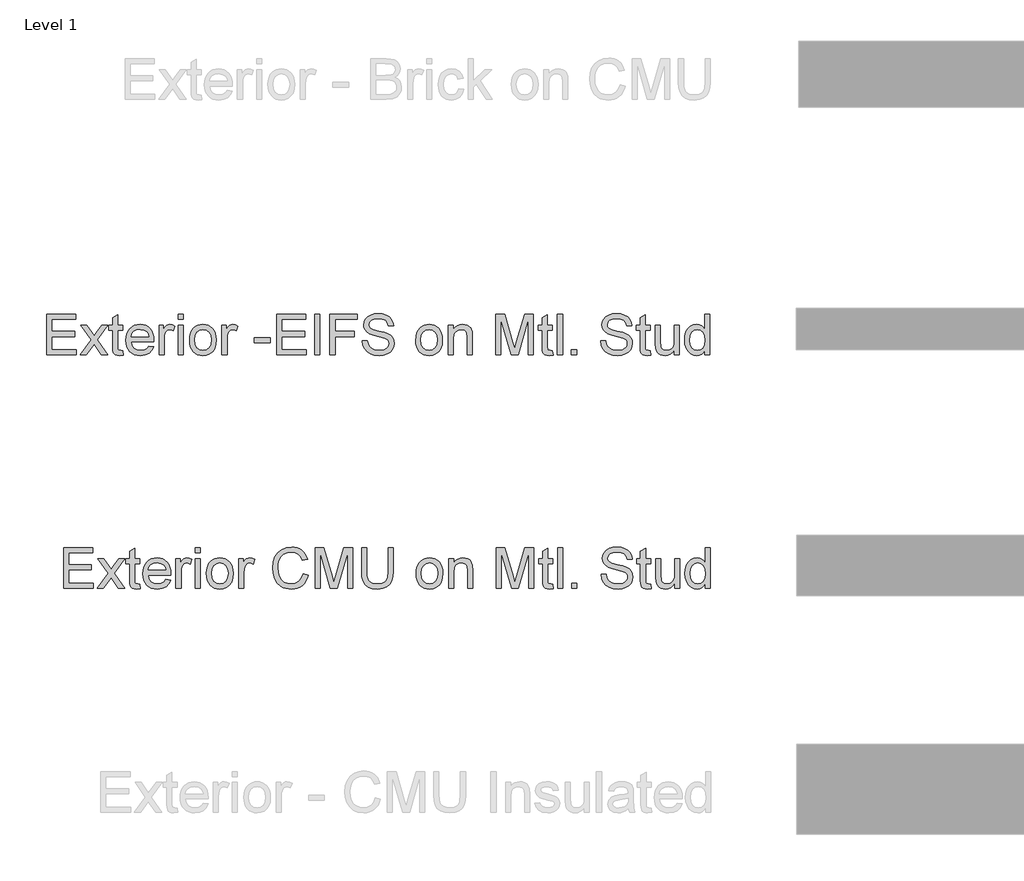
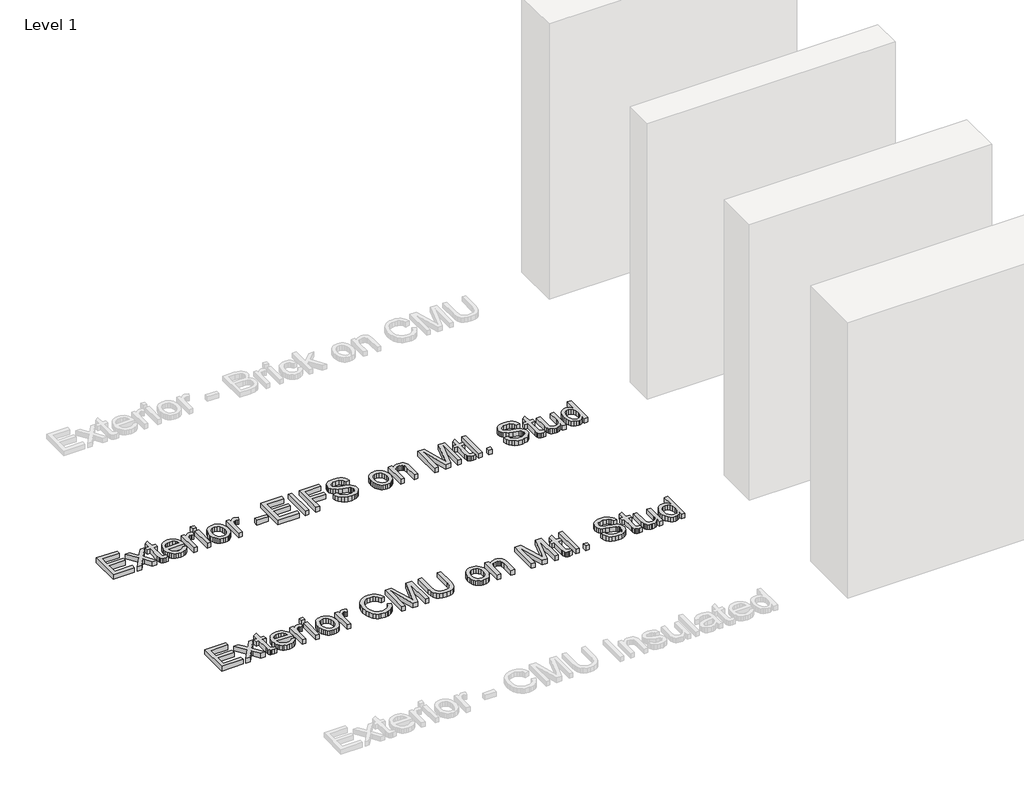
# One storey, part 21 of 42: 2 proxies.
"""IFC4 building model written with IfcOpenShell, lengths in millimetres."""

import ifcopenshell
import ifcopenshell.guid

model = None  # the IFC model being written
_history = None  # IfcOwnerHistory: only IFC2X3 demands one
_inside = {}  # id of a spatial element -> (the spatial element, [elements in it])
_under = {}  # id of a project, library or spatial element -> (it, [spatial elements below it])
_declared = {}  # id of a project -> (the project, [libraries it declares])
_typed = {}  # id of a type object -> (the type object, [elements of that type])
_made_of = {}  # id of a material, layer set ... -> (it, [elements and type objects made of it])


def new_model(schema):
    """Start an empty IFC model of exactly this schema.

    Asked for "IFC4X3", IfcOpenShell would pick the latest addendum, in which some entities
    have other attributes; the version numbers below select the first issue.
    IFC2X3 requires an IfcOwnerHistory on every rooted entity: one is made here for all.
    """
    global model, _history
    if schema == "IFC4X3":
        model = ifcopenshell.file(schema_version=(4, 3, 0, 0))
    else:
        model = ifcopenshell.file(schema=schema)
    _inside.clear()
    _under.clear()
    _declared.clear()
    _typed.clear()
    _made_of.clear()
    _history = None
    if model.schema == "IFC2X3":
        org = make("IfcOrganization", Name="unknown")
        user = make(
            "IfcPersonAndOrganization",
            ThePerson=make("IfcPerson", FamilyName="unknown"),
            TheOrganization=org,
        )
        app = make(
            "IfcApplication",
            ApplicationDeveloper=org,
            Version="unknown",
            ApplicationFullName="unknown",
            ApplicationIdentifier="unknown",
        )
        _history = make(
            "IfcOwnerHistory",
            OwningUser=user,
            OwningApplication=app,
            ChangeAction="ADDED",
            CreationDate=0,
        )
    return model


def make(cls, **values):
    """One entity of the class cls with the attributes given. An attribute that is None is left unset."""
    return model.create_entity(
        cls, **{name: value for name, value in values.items() if value is not None}
    )


def rooted(cls, **values):
    """An entity with a GlobalId (a new one), such as an element, a storey or a relation."""
    return make(cls, GlobalId=ifcopenshell.guid.new(), OwnerHistory=_history, **values)


def si_unit(unit_type, name, prefix=None):
    """IfcSIUnit, for example si_unit("LENGTHUNIT", "METRE", prefix="MILLI")."""
    return make("IfcSIUnit", UnitType=unit_type, Prefix=prefix, Name=name)


def assignment(units):
    """IfcUnitAssignment: the units of a project."""
    return None if units is None else make("IfcUnitAssignment", Units=units)


def point(xyz):
    """IfcCartesianPoint."""
    return None if xyz is None else make("IfcCartesianPoint", Coordinates=xyz)


def direction(xyz):
    """IfcDirection."""
    return None if xyz is None else make("IfcDirection", DirectionRatios=xyz)


def frame(location, z_axis=None, x_axis=None):
    """IfcAxis2Placement3D, a coordinate frame: its origin and axes. An axis left out is left unset."""
    return make(
        "IfcAxis2Placement3D",
        Location=point(location),
        Axis=direction(z_axis),
        RefDirection=direction(x_axis),
    )


def origin():
    """The frame at (0, 0, 0) with its axes left unset."""
    return frame((0.0, 0.0, 0.0))


def origin_with_axes():
    """The frame at (0, 0, 0) with the z axis (0, 0, 1) and the x axis (1, 0, 0) written out."""
    return frame((0.0, 0.0, 0.0), z_axis=(0.0, 0.0, 1.0), x_axis=(1.0, 0.0, 0.0))


def place(relative_to, where):
    """IfcLocalPlacement: puts the frame where relative to a parent placement (None: the world)."""
    return make(
        "IfcLocalPlacement", PlacementRelTo=relative_to, RelativePlacement=where
    )


def context(
    kind, dimensions, precision=None, world=None, true_north=None, identifier=None
):
    """IfcGeometricRepresentationContext, for example the 3D "Model" context."""
    return make(
        "IfcGeometricRepresentationContext",
        ContextIdentifier=identifier,
        ContextType=kind,
        CoordinateSpaceDimension=dimensions,
        Precision=precision,
        WorldCoordinateSystem=world,
        TrueNorth=true_north,
    )


def project(units=None, contexts=None):
    """IfcProject with its units and contexts."""
    return rooted(
        "IfcProject",
        Name="project",
        RepresentationContexts=contexts,
        UnitsInContext=assignment(units),
    )


def spatial(cls, under=None, at=None, **own):
    """A site, building, storey or space (cls), placed at a placement, below another one or the project."""
    s = rooted(cls, ObjectPlacement=at, **own)
    if under is not None:
        _under.setdefault(under.id(), (under, []))[1].append(s)
    return s


def polyline(points):
    """IfcPolyline through the points."""
    return make("IfcPolyline", Points=[point(p) for p in points])


def outline(outer, holes=None, kind="AREA"):
    """IfcArbitraryClosedProfileDef: a profile drawn as a closed curve; with holes, ...WithVoids."""
    if holes is None:
        return make("IfcArbitraryClosedProfileDef", ProfileType=kind, OuterCurve=outer)
    return make(
        "IfcArbitraryProfileDefWithVoids",
        ProfileType=kind,
        OuterCurve=outer,
        InnerCurves=holes,
    )


def extrude(swept, where, along, depth):
    """IfcExtrudedAreaSolid: the profile swept, set in the frame where, extruded along a direction by depth."""
    return make(
        "IfcExtrudedAreaSolid",
        SweptArea=swept,
        Position=where,
        ExtrudedDirection=direction(along),
        Depth=depth,
    )


def shape(context_of_items, identifier, shape_type, items):
    """IfcShapeRepresentation: the items that make up one representation, for example the "Body"."""
    return make(
        "IfcShapeRepresentation",
        ContextOfItems=context_of_items,
        RepresentationIdentifier=identifier,
        RepresentationType=shape_type,
        Items=items,
    )


def made_of(thing, what):
    """Note that an element or type object is made of a material, layer set ...; save() writes the relation."""
    if what is not None:
        _made_of.setdefault(what.id(), (what, []))[1].append(thing)
    return thing


def element(
    cls,
    number,
    at=None,
    inside=None,
    cuts=None,
    type_object=None,
    material=None,
    context=None,
    identifier="Body",
    shape_type=None,
    held_by="IfcProductDefinitionShape",
    body=None,
    shapes=None,
    **own,
):
    """One element of the class cls, such as IfcWall. Its Tag is "e" and its number.

    at: its placement. inside: the storey or other place that contains it. cuts: it is an
    opening in that element (IfcRelVoidsElement). A single representation is given by context,
    identifier, shape_type and body (its items); several are given by shapes. held_by: the class
    of the entity that holds the representations. save() writes the other relations.
    """
    e = rooted(cls, Tag="e%d" % number, ObjectPlacement=at, **own)
    if body is not None:
        shapes = [shape(context, identifier, shape_type, body)]
    if shapes is not None:
        e.Representation = make(held_by, Representations=shapes)
    if inside is not None:
        _inside.setdefault(inside.id(), (inside, []))[1].append(e)
    if cuts is not None:
        rooted(
            "IfcRelVoidsElement", RelatingBuildingElement=cuts, RelatedOpeningElement=e
        )
    if type_object is not None:
        _typed.setdefault(type_object.id(), (type_object, []))[1].append(e)
    return made_of(e, material)


def aggregate(whole, parts):
    """IfcRelAggregates: a whole, such as a stair, and the parts it consists of."""
    return rooted("IfcRelAggregates", RelatingObject=whole, RelatedObjects=parts)


def save(model, path):
    """Write the relations noted so far, then the file.

    IfcRelAggregates (storeys below a building ...), IfcRelContainedInSpatialStructure (elements
    in a storey), IfcRelDefinesByType, IfcRelAssociatesMaterial and IfcRelDeclares: one each for
    every whole, place, type object, material and project.
    """
    for whole, parts in _under.values():
        aggregate(whole, parts)
    for where, things in _inside.values():
        rooted(
            "IfcRelContainedInSpatialStructure",
            RelatedElements=things,
            RelatingStructure=where,
        )
    for kind, things in _typed.values():
        rooted("IfcRelDefinesByType", RelatedObjects=things, RelatingType=kind)
    for what, things in _made_of.values():
        rooted("IfcRelAssociatesMaterial", RelatedObjects=things, RelatingMaterial=what)
    for by, libraries in _declared.values():
        rooted("IfcRelDeclares", RelatingContext=by, RelatedDefinitions=libraries)
    model.write(path)


model = new_model("IFC4")

# Units and contexts
model_context = context("Model", 3, world=origin())
ifc_project = project(units=[si_unit("LENGTHUNIT", "METRE", prefix="MILLI")], contexts=[model_context])

# Site, building, storey
site = spatial("IfcSite", under=ifc_project)
building = spatial("IfcBuilding", under=site)
storey = spatial("IfcBuildingStorey", under=building, Name="Level 1", Elevation=0.0)

# Proxies
placement = place(None, origin())
element("IfcBuildingElementProxy", 1, Name="8\" Arial", ObjectType="8\" Arial", at=placement, inside=storey, context=model_context, shape_type="SweptSolid", body=[
    extrude(outline(polyline([(-4947.8204777, 6427.3124108), (-4947.8204777, 6731.8795049), (-4728.9128788, 6731.8795049), (-4728.9128788, 6693.8086181), (-4909.7495909, 6693.8086181), (-4909.7495909, 6603.390262), (-4738.4306005, 6603.390262), (-4738.4306005, 6565.3193753), (-4909.7495909, 6565.3193753), (-4909.7495909, 6465.3832975), (-4724.154018, 6465.3832975), (-4724.154018, 6427.3124108), (-4947.8204777, 6427.3124108)])), origin_with_axes(), (0.0, 0.0, 1.0), 50.8),
    extrude(outline(polyline([(-4695.6008529, 6427.3124108), (-4614.2540754, 6539.7404982), (-4690.8419921, 6650.9788705), (-4645.0379564, 6650.9788705), (-4608.0824277, 6597.441686), (-4590.8315571, 6572.1602377), (-4575.8857598, 6592.8315395), (-4533.7995842, 6650.9788705), (-4487.9955486, 6650.9788705), (-4568.4500397, 6539.7404982), (-4490.9698366, 6427.3124108), (-4536.7738722, 6427.3124108), (-4583.3958371, 6494.9031062), (-4591.9469151, 6507.2464015), (-4649.7968173, 6427.3124108), (-4695.6008529, 6427.3124108)])), origin_with_axes(), (0.0, 0.0, 1.0), 50.8),
    extrude(outline(polyline([(-4376.7571763, 6459.0629355), (-4371.9983155, 6426.1970528), (-4400.4771233, 6422.5535499), (-4418.7504054, 6424.1336405), (-4432.3763624, 6428.873912), (-4442.0056199, 6436.179507), (-4448.2888034, 6445.4555678), (-4451.7464132, 6461.386598), (-4452.8989498, 6488.6571014), (-4452.8989498, 6612.9079837), (-4481.4521149, 6612.9079837), (-4481.4521149, 6650.9788705), (-4452.8989498, 6650.9788705), (-4452.8989498, 6705.3339842), (-4414.8280631, 6727.7155016), (-4414.8280631, 6650.9788705), (-4376.7571763, 6650.9788705), (-4376.7571763, 6612.9079837), (-4414.8280631, 6612.9079837), (-4414.8280631, 6489.7724594), (-4412.8204187, 6470.1421584), (-4406.3141636, 6463.1897601), (-4393.3388321, 6460.6244367), (-4376.7571763, 6459.0629355)])), origin_with_axes(), (0.0, 0.0, 1.0), 50.8),
    extrude(outline(polyline([(-4182.0900249, 6493.9364626), (-4144.7627101, 6489.1776018), (-4158.2120688, 6461.0519906), (-4179.6734159, 6440.0274921), (-4208.6634295, 6426.9220355), (-4244.6987879, 6422.5535499), (-4268.3211411, 6424.4380402), (-4289.3688762, 6430.0915112), (-4307.8419932, 6439.5139627), (-4323.7404922, 6452.7053948), (-4336.5252834, 6469.2986689), (-4345.6572771, 6488.9266462), (-4351.1364734, 6511.5893268), (-4352.9628721, 6537.2867106), (-4351.1178841, 6563.8554679), (-4345.5829199, 6587.2733388), (-4336.3579797, 6607.5403233), (-4323.4430634, 6624.6564214), (-4307.5863904, 6638.2544945), (-4289.5361799, 6647.9674039), (-4269.292432, 6653.7951495), (-4246.8551467, 6655.7377313), (-4225.1405204, 6653.7997968), (-4205.5032485, 6647.9859932), (-4187.9433308, 6638.2963204), (-4172.4607674, 6624.7307786), (-4159.8223669, 6607.6518591), (-4150.794938, 6587.4220532), (-4145.3784807, 6564.0413609), (-4143.5729949, 6537.5097822), (-4143.7960665, 6527.2484885), (-4314.8919853, 6527.2484885), (-4308.3020784, 6498.7510914), (-4292.9937897, 6477.8009501), (-4270.9004065, 6464.918565), (-4243.9552159, 6460.6244367), (-4223.6928787, 6462.6134918), (-4206.6279011, 6468.5806572), (-4192.7602832, 6478.8977188), (-4182.0900249, 6493.9364626)]), holes=[polyline([(-4314.8919853, 6565.3193753), (-4181.6438817, 6565.3193753), (-4186.7931178, 6585.4329981), (-4196.8871078, 6599.8211164), (-4219.0827322, 6613.2054125), (-4247.0038611, 6617.6668446), (-4272.66639, 6614.1069936), (-4293.8860761, 6603.4274406), (-4308.6366858, 6586.7807223), (-4314.8919853, 6565.3193753)])]), origin_with_axes(), (0.0, 0.0, 1.0), 50.8),
    extrude(outline(polyline([(-4105.5021082, 6427.3124108), (-4105.5021082, 6650.9788705), (-4072.1900823, 6650.9788705), (-4072.1900823, 6617.8899162), (-4059.8839655, 6637.074074), (-4048.5444924, 6648.3763685), (-4037.1678407, 6653.8973906), (-4024.7501882, 6655.7377313), (-4005.789102, 6652.8006219), (-3986.530587, 6643.9892936), (-3999.2456684, 6609.8593385), (-4012.6299645, 6615.7149681), (-4026.0142606, 6617.6668446), (-4037.3816177, 6615.7893253), (-4047.5406702, 6610.1567673), (-4055.7478462, 6601.1967246), (-4061.2595737, 6589.3367511), (-4065.8883095, 6568.0705917), (-4067.4312214, 6544.8711451), (-4067.4312214, 6427.3124108), (-4105.5021082, 6427.3124108)])), origin_with_axes(), (0.0, 0.0, 1.0), 50.8),
    extrude(outline(polyline([(-3962.7362828, 6693.8086181), (-3962.7362828, 6731.8795049), (-3924.6653961, 6731.8795049), (-3924.6653961, 6693.8086181), (-3962.7362828, 6693.8086181)])), origin_with_axes(), (0.0, 0.0, 1.0), 50.8),
    extrude(outline(polyline([(-3962.7362828, 6427.3124108), (-3962.7362828, 6650.9788705), (-3924.6653961, 6650.9788705), (-3924.6653961, 6427.3124108), (-3962.7362828, 6427.3124108)])), origin_with_axes(), (0.0, 0.0, 1.0), 50.8),
    extrude(outline(polyline([(-3877.0767876, 6539.1456406), (-3875.0180226, 6568.1124176), (-3868.8417276, 6593.0732004), (-3858.5479027, 6614.0279891), (-3844.1365477, 6630.9767835), (-3829.6275989, 6641.8096982), (-3813.6129168, 6649.5474944), (-3796.0925014, 6654.1901721), (-3777.0663527, 6655.7377313), (-3756.0627671, 6653.853241), (-3737.0714733, 6648.1997701), (-3720.0924713, 6638.7773186), (-3705.125761, 6625.5858865), (-3692.9102671, 6609.0716169), (-3684.1849143, 6589.6806532), (-3678.9497027, 6567.4129952), (-3677.2046321, 6542.2686431), (-3680.290456, 6503.807381), (-3689.5479274, 6474.5292332), (-3704.7075017, 6452.6031537), (-3725.499634, 6436.1980963), (-3750.1955193, 6425.9646865), (-3777.0663527, 6422.5535499), (-3798.3766617, 6424.4310693), (-3817.5445538, 6430.0636272), (-3834.5700291, 6439.4512238), (-3849.4530876, 6452.593859), (-3861.5384563, 6469.2684613), (-3870.1708626, 6489.251959), (-3875.3503064, 6512.5443521), (-3877.0767876, 6539.1456406)]), holes=[polyline([(-3839.0059009, 6539.2199978), (-3834.6002367, 6504.76473), (-3821.3832443, 6480.2175591), (-3801.4926931, 6465.5227173), (-3777.0663527, 6460.6244367), (-3752.751548, 6465.5506012), (-3732.8981755, 6480.3290949), (-3719.681183, 6505.2015785), (-3715.2755189, 6540.409713), (-3719.709067, 6573.8611587), (-3733.0097113, 6598.0737222), (-3752.8909678, 6612.768564), (-3777.0663527, 6617.6668446), (-3801.4926931, 6612.7871533), (-3821.3832443, 6598.1480794), (-3834.6002367, 6573.6566764), (-3839.0059009, 6539.2199978)])]), origin_with_axes(), (0.0, 0.0, 1.0), 50.8),
    extrude(outline(polyline([(-3634.3748845, 6427.3124108), (-3634.3748845, 6650.9788705), (-3601.0628586, 6650.9788705), (-3601.0628586, 6617.8899162), (-3588.7567419, 6637.074074), (-3577.4172688, 6648.3763685), (-3566.0406171, 6653.8973906), (-3553.6229646, 6655.7377313), (-3534.6618784, 6652.8006219), (-3515.4033634, 6643.9892936), (-3528.1184447, 6609.8593385), (-3541.5027409, 6615.7149681), (-3554.887037, 6617.6668446), (-3566.254394, 6615.7893253), (-3576.4134466, 6610.1567673), (-3584.6206226, 6601.1967246), (-3590.1323501, 6589.3367511), (-3594.7610859, 6568.0705917), (-3596.3039978, 6544.8711451), (-3596.3039978, 6427.3124108), (-3634.3748845, 6427.3124108)])), origin_with_axes(), (0.0, 0.0, 1.0), 50.8),
    extrude(outline(polyline([(-3391.6729814, 6517.7307668), (-3391.6729814, 6555.8016536), (-3272.7014603, 6555.8016536), (-3272.7014603, 6517.7307668), (-3391.6729814, 6517.7307668)])), origin_with_axes(), (0.0, 0.0, 1.0), 50.8),
    extrude(outline(polyline([(-3225.1128519, 6427.3124108), (-3225.1128519, 6731.8795049), (-3006.205253, 6731.8795049), (-3006.205253, 6693.8086181), (-3187.0419651, 6693.8086181), (-3187.0419651, 6603.390262), (-3015.7229747, 6603.390262), (-3015.7229747, 6565.3193753), (-3187.0419651, 6565.3193753), (-3187.0419651, 6465.3832975), (-3001.4463922, 6465.3832975), (-3001.4463922, 6427.3124108), (-3225.1128519, 6427.3124108)])), origin_with_axes(), (0.0, 0.0, 1.0), 50.8),
    extrude(outline(polyline([(-2939.5812012, 6427.3124108), (-2939.5812012, 6731.8795049), (-2901.5103144, 6731.8795049), (-2901.5103144, 6427.3124108), (-2939.5812012, 6427.3124108)])), origin_with_axes(), (0.0, 0.0, 1.0), 50.8),
    extrude(outline(polyline([(-2825.3685409, 6427.3124108), (-2825.3685409, 6731.8795049), (-2620.7375246, 6731.8795049), (-2620.7375246, 6693.8086181), (-2787.2976542, 6693.8086181), (-2787.2976542, 6603.390262), (-2644.5318288, 6603.390262), (-2644.5318288, 6565.3193753), (-2787.2976542, 6565.3193753), (-2787.2976542, 6427.3124108), (-2825.3685409, 6427.3124108)])), origin_with_axes(), (0.0, 0.0, 1.0), 50.8),
    extrude(outline(polyline([(-2582.6666378, 6532.0073494), (-2544.5957511, 6532.0073494), (-2540.2272655, 6510.8806097), (-2532.3268129, 6493.899284), (-2520.0021069, 6480.4220414), (-2502.3608611, 6469.807551), (-2480.7972729, 6462.9202153), (-2456.7055398, 6460.6244367), (-2435.4951483, 6462.3625363), (-2416.9244375, 6467.576835), (-2401.876399, 6475.8304842), (-2391.2340246, 6486.6866355), (-2384.9043679, 6499.1507613), (-2382.7944823, 6512.228334), (-2384.3745729, 6524.9712993), (-2389.1148444, 6535.9854596), (-2398.7441019, 6545.3823508), (-2414.9911502, 6553.2735088), (-2470.4244434, 6567.8103415), (-2506.8129985, 6577.4303043), (-2530.0960969, 6586.5855347), (-2549.0478885, 6599.3935625), (-2562.4786578, 6614.9156281), (-2570.4813516, 6632.8171242), (-2573.1489161, 6652.7634433), (-2569.8493154, 6675.0613089), (-2559.950513, 6695.8534411), (-2543.7127593, 6713.4760977), (-2521.3963044, 6726.2655362), (-2494.6091229, 6734.0451583), (-2464.9591891, 6736.6383657), (-2432.8368784, 6733.9243279), (-2404.7298565, 6725.7822144), (-2381.6419457, 6712.379329), (-2364.5769682, 6693.8829753), (-2353.7765848, 6671.44569), (-2349.4824564, 6646.2200096), (-2387.5533432, 6646.2200096), (-2394.5429201, 6668.9361345), (-2409.1169314, 6685.3318972), (-2431.8888241, 6695.2585835), (-2463.4720451, 6698.5674789), (-2495.7988381, 6695.2957621), (-2517.9758732, 6685.4806116), (-2530.8024903, 6671.0367254), (-2535.0780294, 6653.8788013), (-2532.0479734, 6639.2490221), (-2522.9578057, 6627.4819951), (-2501.4685747, 6616.9604512), (-2460.7951859, 6606.2158357), (-2418.8205461, 6596.0103099), (-2393.427562, 6587.1060351), (-2371.7245541, 6573.2941851), (-2356.5835691, 6556.2477968), (-2347.688589, 6536.1527633), (-2344.7235956, 6513.1949776), (-2348.1347322, 6489.7259861), (-2358.3681419, 6467.6511922), (-2375.0055656, 6448.6529274), (-2397.6287439, 6434.4135234), (-2424.8341847, 6425.5185433), (-2455.2183958, 6422.5535499), (-2492.5178266, 6425.7509096), (-2523.2180559, 6435.3429885), (-2547.6722802, 6451.3669652), (-2566.2336965, 6473.8600184), (-2578.1494379, 6501.2606469), (-2582.6666378, 6532.0073494)])), origin_with_axes(), (0.0, 0.0, 1.0), 50.8),
    extrude(outline(polyline([(-2182.9223269, 6539.1456406), (-2180.8635619, 6568.1124176), (-2174.6872669, 6593.0732004), (-2164.3934419, 6614.0279891), (-2149.9820869, 6630.9767835), (-2135.4731382, 6641.8096982), (-2119.4584561, 6649.5474944), (-2101.9380406, 6654.1901721), (-2082.9118919, 6655.7377313), (-2061.9083064, 6653.853241), (-2042.9170126, 6648.1997701), (-2025.9380105, 6638.7773186), (-2010.9713002, 6625.5858865), (-1998.7558064, 6609.0716169), (-1990.0304536, 6589.6806532), (-1984.7952419, 6567.4129952), (-1983.0501714, 6542.2686431), (-1986.1359952, 6503.807381), (-1995.3934667, 6474.5292332), (-2010.553041, 6452.6031537), (-2031.3451732, 6436.1980963), (-2056.0410585, 6425.9646865), (-2082.9118919, 6422.5535499), (-2104.2222009, 6424.4310693), (-2123.390093, 6430.0636272), (-2140.4155683, 6439.4512238), (-2155.2986268, 6452.593859), (-2167.3839956, 6469.2684613), (-2176.0164018, 6489.251959), (-2181.1958456, 6512.5443521), (-2182.9223269, 6539.1456406)]), holes=[polyline([(-2144.8514401, 6539.2199978), (-2140.445776, 6504.76473), (-2127.2287835, 6480.2175591), (-2107.3382323, 6465.5227173), (-2082.9118919, 6460.6244367), (-2058.5970873, 6465.5506012), (-2038.7437147, 6480.3290949), (-2025.5267223, 6505.2015785), (-2021.1210581, 6540.409713), (-2025.5546062, 6573.8611587), (-2038.8552505, 6598.0737222), (-2058.736507, 6612.768564), (-2082.9118919, 6617.6668446), (-2107.3382323, 6612.7871533), (-2127.2287835, 6598.1480794), (-2140.445776, 6573.6566764), (-2144.8514401, 6539.2199978)])]), origin_with_axes(), (0.0, 0.0, 1.0), 50.8),
    extrude(outline(polyline([(-1940.2204238, 6427.3124108), (-1940.2204238, 6650.9788705), (-1902.149537, 6650.9788705), (-1902.149537, 6619.7488462), (-1888.9232499, 6635.4939834), (-1873.0386929, 6646.74051), (-1854.495866, 6653.488426), (-1833.2947692, 6655.7377313), (-1814.5288706, 6653.9252746), (-1797.3430626, 6648.4879043), (-1783.0107122, 6640.1041299), (-1772.8051864, 6629.4524609), (-1761.3913561, 6601.4569748), (-1759.3837117, 6564.6501605), (-1759.3837117, 6427.3124108), (-1797.4545984, 6427.3124108), (-1797.4545984, 6559.5195136), (-1801.8416733, 6593.2033255), (-1807.9110798, 6603.232253), (-1817.3451496, 6611.0118751), (-1829.4374894, 6616.0031022), (-1843.4817057, 6617.6668446), (-1865.7795712, 6613.9303952), (-1884.7871307, 6602.7210472), (-1892.3831834, 6593.5704642), (-1897.8089354, 6581.0645125), (-1902.149537, 6545.9865031), (-1902.149537, 6427.3124108), (-1940.2204238, 6427.3124108)])), origin_with_axes(), (0.0, 0.0, 1.0), 50.8),
    extrude(outline(polyline([(-1583.3058604, 6427.3124108), (-1583.3058604, 6731.8795049), (-1517.7971666, 6731.8795049), (-1455.4858324, 6517.2102664), (-1442.9194655, 6472.3728744), (-1429.3120978, 6520.9281265), (-1368.0417644, 6731.8795049), (-1302.5330706, 6731.8795049), (-1302.5330706, 6427.3124108), (-1340.6039573, 6427.3124108), (-1340.6039573, 6693.8086181), (-1417.1175168, 6427.3124108), (-1468.7214141, 6427.3124108), (-1545.2349737, 6693.8086181), (-1545.2349737, 6427.3124108), (-1583.3058604, 6427.3124108)])), origin_with_axes(), (0.0, 0.0, 1.0), 50.8),
    extrude(outline(polyline([(-1159.7672452, 6459.0629355), (-1155.0083844, 6426.1970528), (-1183.4871922, 6422.5535499), (-1201.7604743, 6424.1336405), (-1215.3864313, 6428.873912), (-1225.0156888, 6436.179507), (-1231.2988723, 6445.4555678), (-1234.7564821, 6461.386598), (-1235.9090187, 6488.6571014), (-1235.9090187, 6612.9079837), (-1264.4621838, 6612.9079837), (-1264.4621838, 6650.9788705), (-1235.9090187, 6650.9788705), (-1235.9090187, 6705.3339842), (-1197.838132, 6727.7155016), (-1197.838132, 6650.9788705), (-1159.7672452, 6650.9788705), (-1159.7672452, 6612.9079837), (-1197.838132, 6612.9079837), (-1197.838132, 6489.7724594), (-1195.8304876, 6470.1421584), (-1189.3242325, 6463.1897601), (-1176.348901, 6460.6244367), (-1159.7672452, 6459.0629355)])), origin_with_axes(), (0.0, 0.0, 1.0), 50.8),
    extrude(outline(polyline([(-1121.6963585, 6427.3124108), (-1121.6963585, 6731.8795049), (-1083.6254717, 6731.8795049), (-1083.6254717, 6427.3124108), (-1121.6963585, 6427.3124108)])), origin_with_axes(), (0.0, 0.0, 1.0), 50.8),
    extrude(outline(polyline([(-1017.0014199, 6427.3124108), (-1017.0014199, 6465.3832975), (-978.9305331, 6465.3832975), (-978.9305331, 6427.3124108), (-1017.0014199, 6427.3124108)])), origin_with_axes(), (0.0, 0.0, 1.0), 50.8),
    extrude(outline(polyline([(-798.093821, 6532.0073494), (-760.0229343, 6532.0073494), (-755.6544487, 6510.8806097), (-747.7539961, 6493.899284), (-735.4292901, 6480.4220414), (-717.7880443, 6469.807551), (-696.2244561, 6462.9202153), (-672.132723, 6460.6244367), (-650.9223315, 6462.3625363), (-632.3516207, 6467.576835), (-617.3035822, 6475.8304842), (-606.6612078, 6486.6866355), (-600.3315511, 6499.1507613), (-598.2216655, 6512.228334), (-599.801756, 6524.9712993), (-604.5420276, 6535.9854596), (-614.1712851, 6545.3823508), (-630.4183334, 6553.2735088), (-685.8516266, 6567.8103415), (-722.2401817, 6577.4303043), (-745.5232801, 6586.5855347), (-764.4750717, 6599.3935625), (-777.905841, 6614.9156281), (-785.9085348, 6632.8171242), (-788.5760993, 6652.7634433), (-785.2764985, 6675.0613089), (-775.3776962, 6695.8534411), (-759.1399425, 6713.4760977), (-736.8234876, 6726.2655362), (-710.0363061, 6734.0451583), (-680.3863723, 6736.6383657), (-648.2640616, 6733.9243279), (-620.1570397, 6725.7822144), (-597.0691289, 6712.379329), (-580.0041514, 6693.8829753), (-569.203768, 6671.44569), (-564.9096396, 6646.2200096), (-602.9805264, 6646.2200096), (-609.9701032, 6668.9361345), (-624.5441146, 6685.3318972), (-647.3160073, 6695.2585835), (-678.8992283, 6698.5674789), (-711.2260213, 6695.2957621), (-733.4030564, 6685.4806116), (-746.2296735, 6671.0367254), (-750.5052126, 6653.8788013), (-747.4751566, 6639.2490221), (-738.3849889, 6627.4819951), (-716.8957579, 6616.9604512), (-676.2223691, 6606.2158357), (-634.2477293, 6596.0103099), (-608.8547452, 6587.1060351), (-587.1517373, 6573.2941851), (-572.0107523, 6556.2477968), (-563.1157722, 6536.1527633), (-560.1507788, 6513.1949776), (-563.5619154, 6489.7259861), (-573.7953251, 6467.6511922), (-590.4327488, 6448.6529274), (-613.0559271, 6434.4135234), (-640.2613679, 6425.5185433), (-670.645579, 6422.5535499), (-707.9450098, 6425.7509096), (-738.6452391, 6435.3429885), (-763.0994634, 6451.3669652), (-781.6608797, 6473.8600184), (-793.5766211, 6501.2606469), (-798.093821, 6532.0073494)])), origin_with_axes(), (0.0, 0.0, 1.0), 50.8),
    extrude(outline(polyline([(-426.9026751, 6459.0629355), (-422.1438143, 6426.1970528), (-450.6226221, 6422.5535499), (-468.8959042, 6424.1336405), (-482.5218612, 6428.873912), (-492.1511187, 6436.179507), (-498.4343022, 6445.4555678), (-501.891912, 6461.386598), (-503.0444486, 6488.6571014), (-503.0444486, 6612.9079837), (-531.5976137, 6612.9079837), (-531.5976137, 6650.9788705), (-503.0444486, 6650.9788705), (-503.0444486, 6705.3339842), (-464.9735619, 6727.7155016), (-464.9735619, 6650.9788705), (-426.9026751, 6650.9788705), (-426.9026751, 6612.9079837), (-464.9735619, 6612.9079837), (-464.9735619, 6489.7724594), (-462.9659175, 6470.1421584), (-456.4596624, 6463.1897601), (-443.4843309, 6460.6244367), (-426.9026751, 6459.0629355)])), origin_with_axes(), (0.0, 0.0, 1.0), 50.8),
    extrude(outline(polyline([(-246.065963, 6427.3124108), (-246.065963, 6465.7550835), (-259.8406344, 6446.8544126), (-275.8832005, 6433.3539333), (-294.1936612, 6425.2536458), (-314.7720165, 6422.5535499), (-333.3148434, 6424.4496586), (-350.5750086, 6430.1379844), (-365.0560734, 6438.6890625), (-375.2615992, 6449.1734278), (-382.1303456, 6461.9070984), (-386.6010723, 6477.2060925), (-388.8317884, 6512.60012), (-388.8317884, 6650.9788705), (-350.7609016, 6650.9788705), (-350.7609016, 6530.5202054), (-348.4558284, 6491.7057466), (-342.9069223, 6478.758299), (-333.3984952, 6468.9152646), (-320.5625835, 6462.6971437), (-305.0312232, 6460.6244367), (-288.6075765, 6462.7436169), (-273.2435199, 6469.1011576), (-260.5749118, 6479.1114957), (-252.2376107, 6492.1890684), (-247.6088749, 6510.0998591), (-246.065963, 6534.6098514), (-246.065963, 6650.9788705), (-207.9950763, 6650.9788705), (-207.9950763, 6427.3124108), (-246.065963, 6427.3124108)])), origin_with_axes(), (0.0, 0.0, 1.0), 50.8),
    extrude(outline(polyline([(-17.6406425, 6427.3124108), (-17.6406425, 6463.2269387), (-29.0312361, 6445.4323311), (-42.8291442, 6432.7218971), (-59.0343666, 6425.0956367), (-77.6469034, 6422.5535499), (-102.2591369, 6426.2342314), (-124.7893687, 6437.2762757), (-143.8619907, 6454.9082269), (-158.1013946, 6478.3586291), (-166.9684908, 6506.6794279), (-169.9241895, 6538.922569), (-167.200857, 6570.7660402), (-159.0308596, 6599.5236876), (-145.4234919, 6623.5596527), (-126.3880485, 6641.2380772), (-103.3652002, 6652.1128178), (-77.7956178, 6655.7377313), (-59.1691391, 6653.144524), (-42.6990191, 6645.3649018), (-28.7384547, 6633.4398658), (-17.6406425, 6618.4104166), (-17.6406425, 6731.8795049), (20.4302443, 6731.8795049), (20.4302443, 6427.3124108), (-17.6406425, 6427.3124108)]), holes=[polyline([(-131.8533027, 6539.0712834), (-127.5591744, 6504.6346049), (-114.6767894, 6480.1432019), (-95.9573641, 6465.504128), (-74.152115, 6460.6244367), (-52.3561605, 6465.2810564), (-34.1107624, 6479.2509155), (-21.7581725, 6502.7942641), (-17.6406425, 6536.1713526), (-21.8325297, 6572.6621489), (-34.4081912, 6597.9621864), (-53.1183219, 6612.74068), (-75.7136162, 6617.6668446), (-97.7419369, 6612.9358677), (-115.7921474, 6598.742937), (-127.8380139, 6574.3630698), (-131.8533027, 6539.0712834)])]), origin_with_axes(), (0.0, 0.0, 1.0), 50.8),
])
element("IfcBuildingElementProxy", 2, Name="8\" Arial", ObjectType="8\" Arial", at=placement, inside=storey, context=model_context, shape_type="SweptSolid", body=[
    extrude(outline(polyline([(-4820.8204777, 4678.9650607), (-4820.8204777, 4983.5321548), (-4601.9128788, 4983.5321548), (-4601.9128788, 4945.461268), (-4782.7495909, 4945.461268), (-4782.7495909, 4855.042912), (-4611.4306005, 4855.042912), (-4611.4306005, 4816.9720252), (-4782.7495909, 4816.9720252), (-4782.7495909, 4717.0359475), (-4597.154018, 4717.0359475), (-4597.154018, 4678.9650607), (-4820.8204777, 4678.9650607)])), origin_with_axes(), (0.0, 0.0, 1.0), 50.8),
    extrude(outline(polyline([(-4568.6008529, 4678.9650607), (-4487.2540754, 4791.3931482), (-4563.8419921, 4902.6315204), (-4518.0379564, 4902.6315204), (-4481.0824277, 4849.0943359), (-4463.8315571, 4823.8128877), (-4448.8857598, 4844.4841895), (-4406.7995842, 4902.6315204), (-4360.9955486, 4902.6315204), (-4441.4500397, 4791.3931482), (-4363.9698366, 4678.9650607), (-4409.7738722, 4678.9650607), (-4456.3958371, 4746.5557562), (-4464.9469151, 4758.8990515), (-4522.7968173, 4678.9650607), (-4568.6008529, 4678.9650607)])), origin_with_axes(), (0.0, 0.0, 1.0), 50.8),
    extrude(outline(polyline([(-4249.7571763, 4710.7155854), (-4244.9983155, 4677.8497027), (-4273.4771233, 4674.2061999), (-4291.7504054, 4675.7862904), (-4305.3763624, 4680.526562), (-4315.0056199, 4687.8321569), (-4321.2888034, 4697.1082177), (-4324.7464132, 4713.039248), (-4325.8989498, 4740.3097513), (-4325.8989498, 4864.5606337), (-4354.4521149, 4864.5606337), (-4354.4521149, 4902.6315204), (-4325.8989498, 4902.6315204), (-4325.8989498, 4956.9866342), (-4287.8280631, 4979.3681516), (-4287.8280631, 4902.6315204), (-4249.7571763, 4902.6315204), (-4249.7571763, 4864.5606337), (-4287.8280631, 4864.5606337), (-4287.8280631, 4741.4251093), (-4285.8204187, 4721.7948083), (-4279.3141636, 4714.8424101), (-4266.3388321, 4712.2770867), (-4249.7571763, 4710.7155854)])), origin_with_axes(), (0.0, 0.0, 1.0), 50.8),
    extrude(outline(polyline([(-4055.0900249, 4745.5891126), (-4017.7627101, 4740.8302517), (-4031.2120688, 4712.7046406), (-4052.6734159, 4691.6801421), (-4081.6634295, 4678.5746854), (-4117.6987879, 4674.2061999), (-4141.3211411, 4676.0906902), (-4162.3688762, 4681.7441611), (-4180.8419932, 4691.1666126), (-4196.7404922, 4704.3580448), (-4209.5252834, 4720.9513188), (-4218.6572771, 4740.5792962), (-4224.1364734, 4763.2419767), (-4225.9628721, 4788.9393606), (-4224.1178841, 4815.5081179), (-4218.5829199, 4838.9259887), (-4209.3579797, 4859.1929733), (-4196.4430634, 4876.3090714), (-4180.5863904, 4889.9071445), (-4162.5361799, 4899.6200538), (-4142.292432, 4905.4477994), (-4119.8551467, 4907.3903813), (-4098.1405204, 4905.4524467), (-4078.5032485, 4899.6386431), (-4060.9433308, 4889.9489704), (-4045.4607674, 4876.3834286), (-4032.8223669, 4859.3045091), (-4023.794938, 4839.0747031), (-4018.3784807, 4815.6940109), (-4016.5729949, 4789.1624322), (-4016.7960665, 4778.9011385), (-4187.8919853, 4778.9011385), (-4181.3020784, 4750.4037413), (-4165.9937897, 4729.4536), (-4143.9004065, 4716.571215), (-4116.9552159, 4712.2770867), (-4096.6928787, 4714.2661418), (-4079.6279011, 4720.2333071), (-4065.7602832, 4730.5503687), (-4055.0900249, 4745.5891126)]), holes=[polyline([(-4187.8919853, 4816.9720252), (-4054.6438817, 4816.9720252), (-4059.7931178, 4837.085648), (-4069.8871078, 4851.4737664), (-4092.0827322, 4864.8580625), (-4120.0038611, 4869.3194945), (-4145.66639, 4865.7596435), (-4166.8860761, 4855.0800906), (-4181.6366858, 4838.4333723), (-4187.8919853, 4816.9720252)])]), origin_with_axes(), (0.0, 0.0, 1.0), 50.8),
    extrude(outline(polyline([(-3978.5021082, 4678.9650607), (-3978.5021082, 4902.6315204), (-3945.1900823, 4902.6315204), (-3945.1900823, 4869.5425661), (-3932.8839655, 4888.7267239), (-3921.5444924, 4900.0290184), (-3910.1678407, 4905.5500406), (-3897.7501882, 4907.3903813), (-3878.789102, 4904.4532719), (-3859.530587, 4895.6419436), (-3872.2456684, 4861.5119885), (-3885.6299645, 4867.367618), (-3899.0142606, 4869.3194945), (-3910.3816177, 4867.4419752), (-3920.5406702, 4861.8094173), (-3928.7478462, 4852.8493746), (-3934.2595737, 4840.9894011), (-3938.8883095, 4819.7232417), (-3940.4312214, 4796.523795), (-3940.4312214, 4678.9650607), (-3978.5021082, 4678.9650607)])), origin_with_axes(), (0.0, 0.0, 1.0), 50.8),
    extrude(outline(polyline([(-3835.7362828, 4945.461268), (-3835.7362828, 4983.5321548), (-3797.6653961, 4983.5321548), (-3797.6653961, 4945.461268), (-3835.7362828, 4945.461268)])), origin_with_axes(), (0.0, 0.0, 1.0), 50.8),
    extrude(outline(polyline([(-3835.7362828, 4678.9650607), (-3835.7362828, 4902.6315204), (-3797.6653961, 4902.6315204), (-3797.6653961, 4678.9650607), (-3835.7362828, 4678.9650607)])), origin_with_axes(), (0.0, 0.0, 1.0), 50.8),
    extrude(outline(polyline([(-3750.0767876, 4790.7982906), (-3748.0180226, 4819.7650676), (-3741.8417276, 4844.7258504), (-3731.5479027, 4865.680639), (-3717.1365477, 4882.6294335), (-3702.6275989, 4893.4623481), (-3686.6129168, 4901.2001443), (-3669.0925014, 4905.8428221), (-3650.0663527, 4907.3903813), (-3629.0627671, 4905.505891), (-3610.0714733, 4899.8524201), (-3593.0924713, 4890.4299685), (-3578.125761, 4877.2385364), (-3565.9102671, 4860.7242669), (-3557.1849143, 4841.3333031), (-3551.9497027, 4819.0656452), (-3550.2046321, 4793.921293), (-3553.290456, 4755.460031), (-3562.5479274, 4726.1818832), (-3577.7075017, 4704.2558036), (-3598.499634, 4687.8507462), (-3623.1955193, 4677.6173365), (-3650.0663527, 4674.2061999), (-3671.3766617, 4676.0837192), (-3690.5445538, 4681.7162772), (-3707.5700291, 4691.1038738), (-3722.4530876, 4704.246509), (-3734.5384563, 4720.9211112), (-3743.1708626, 4740.9046089), (-3748.3503064, 4764.197002), (-3750.0767876, 4790.7982906)]), holes=[polyline([(-3712.0059009, 4790.8726478), (-3707.6002367, 4756.4173799), (-3694.3832443, 4731.870209), (-3674.4926931, 4717.1753672), (-3650.0663527, 4712.2770867), (-3625.751548, 4717.2032512), (-3605.8981755, 4731.9817448), (-3592.681183, 4756.8542285), (-3588.2755189, 4792.062363), (-3592.709067, 4825.5138087), (-3606.0097113, 4849.7263721), (-3625.8909678, 4864.4212139), (-3650.0663527, 4869.3194945), (-3674.4926931, 4864.4398032), (-3694.3832443, 4849.8007293), (-3707.6002367, 4825.3093264), (-3712.0059009, 4790.8726478)])]), origin_with_axes(), (0.0, 0.0, 1.0), 50.8),
    extrude(outline(polyline([(-3507.3748845, 4678.9650607), (-3507.3748845, 4902.6315204), (-3474.0628586, 4902.6315204), (-3474.0628586, 4869.5425661), (-3461.7567419, 4888.7267239), (-3450.4172688, 4900.0290184), (-3439.0406171, 4905.5500406), (-3426.6229646, 4907.3903813), (-3407.6618784, 4904.4532719), (-3388.4033634, 4895.6419436), (-3401.1184447, 4861.5119885), (-3414.5027409, 4867.367618), (-3427.887037, 4869.3194945), (-3439.254394, 4867.4419752), (-3449.4134466, 4861.8094173), (-3457.6206226, 4852.8493746), (-3463.1323501, 4840.9894011), (-3467.7610859, 4819.7232417), (-3469.3039978, 4796.523795), (-3469.3039978, 4678.9650607), (-3507.3748845, 4678.9650607)])), origin_with_axes(), (0.0, 0.0, 1.0), 50.8),
    extrude(outline(polyline([(-3026.7299392, 4787.229145), (-2988.6590524, 4777.4139945), (-2996.1923663, 4753.738197), (-3006.2259411, 4733.0506296), (-3018.7597768, 4715.3512922), (-3033.7938733, 4700.6401847), (-3050.9889759, 4689.0753164), (-3070.00583, 4680.8146961), (-3090.8444355, 4675.8583239), (-3113.5047924, 4674.2061999), (-3157.663675, 4679.2067216), (-3176.3343033, 4685.4573738), (-3192.7323898, 4694.2082869), (-3219.6125178, 4718.6903952), (-3239.2056402, 4752.1325462), (-3251.1678549, 4791.4489161), (-3255.1552598, 4833.553681), (-3250.6473545, 4877.9635191), (-3237.1236386, 4916.3132454), (-3215.2905055, 4947.3852606), (-3185.8543487, 4969.9619657), (-3150.943643, 4983.7087532), (-3112.6868632, 4988.2910157), (-3090.9118217, 4986.808519), (-3070.9445897, 4982.3610289), (-3052.7851671, 4974.9485455), (-3036.4335539, 4964.5710686), (-3022.159295, 4951.5027906), (-3010.2319353, 4936.0179036), (-2993.4179133, 4897.7983024), (-3031.4888, 4888.7267239), (-3044.6872032, 4916.4898437), (-3062.7188243, 4935.5345818), (-3085.8067352, 4946.5487421), (-3114.1740072, 4950.2201289), (-3146.8725862, 4946.1490722), (-3173.734125, 4933.9359019), (-3194.1172926, 4914.86328), (-3207.3807583, 4890.2138679), (-3214.6584693, 4862.348507), (-3217.084373, 4833.6280382), (-3214.2123261, 4798.4570823), (-3205.5961855, 4768.0449872), (-3190.9106383, 4743.5535842), (-3169.8303719, 4726.1447046), (-3144.5582184, 4715.7439911), (-3117.2970097, 4712.2770867), (-3085.518601, 4716.9987689), (-3059.0381429, 4731.1638156), (-3039.0453506, 4754.6235125), (-3026.7299392, 4787.229145)])), origin_with_axes(), (0.0, 0.0, 1.0), 50.8),
    extrude(outline(polyline([(-2936.3115831, 4678.9650607), (-2936.3115831, 4983.5321548), (-2870.8028893, 4983.5321548), (-2808.4915551, 4768.8629164), (-2795.9251882, 4724.0255244), (-2782.3178205, 4772.5807764), (-2721.0474871, 4983.5321548), (-2655.5387933, 4983.5321548), (-2655.5387933, 4678.9650607), (-2693.6096801, 4678.9650607), (-2693.6096801, 4945.461268), (-2770.1232396, 4678.9650607), (-2821.7271369, 4678.9650607), (-2898.2406964, 4945.461268), (-2898.2406964, 4678.9650607), (-2936.3115831, 4678.9650607)])), origin_with_axes(), (0.0, 0.0, 1.0), 50.8),
    extrude(outline(polyline([(-2389.042586, 4983.5321548), (-2350.9716992, 4983.5321548), (-2350.9716992, 4807.8260896), (-2353.555612, 4766.6786736), (-2361.3073501, 4734.9932115), (-2375.788415, 4710.5482817), (-2398.5603077, 4691.1224631), (-2429.6787962, 4678.4352657), (-2469.1996484, 4674.2061999), (-2507.8560981, 4677.8868813), (-2538.7608096, 4688.9289256), (-2561.9230776, 4706.9512522), (-2577.3521968, 4731.5727802), (-2586.0241053, 4764.596672), (-2588.9147415, 4807.8260896), (-2588.9147415, 4983.5321548), (-2550.8438547, 4983.5321548), (-2550.8438547, 4809.1645192), (-2548.9663354, 4774.9509122), (-2543.3337774, 4751.128724), (-2533.1282517, 4734.6307201), (-2517.5318288, 4722.3896659), (-2497.1951344, 4714.8052315), (-2472.768794, 4712.2770867), (-2434.0472817, 4717.2776084), (-2419.5522749, 4723.5282606), (-2408.301101, 4732.2791736), (-2399.8755007, 4744.5852904), (-2393.8572147, 4761.5015535), (-2389.042586, 4809.1645192), (-2389.042586, 4983.5321548)])), origin_with_axes(), (0.0, 0.0, 1.0), 50.8),
    extrude(outline(polyline([(-2179.6527088, 4790.7982906), (-2177.5939438, 4819.7650676), (-2171.4176488, 4844.7258504), (-2161.1238239, 4865.680639), (-2146.7124689, 4882.6294335), (-2132.2035201, 4893.4623481), (-2116.188838, 4901.2001443), (-2098.6684226, 4905.8428221), (-2079.6422739, 4907.3903813), (-2058.6386883, 4905.505891), (-2039.6473946, 4899.8524201), (-2022.6683925, 4890.4299685), (-2007.7016822, 4877.2385364), (-1995.4861883, 4860.7242669), (-1986.7608356, 4841.3333031), (-1981.5256239, 4819.0656452), (-1979.7805533, 4793.921293), (-1982.8663772, 4755.460031), (-1992.1238487, 4726.1818832), (-2007.283423, 4704.2558036), (-2028.0755552, 4687.8507462), (-2052.7714405, 4677.6173365), (-2079.6422739, 4674.2061999), (-2100.9525829, 4676.0837192), (-2120.120475, 4681.7162772), (-2137.1459503, 4691.1038738), (-2152.0290088, 4704.246509), (-2164.1143775, 4720.9211112), (-2172.7467838, 4740.9046089), (-2177.9262276, 4764.197002), (-2179.6527088, 4790.7982906)]), holes=[polyline([(-2141.5818221, 4790.8726478), (-2137.1761579, 4756.4173799), (-2123.9591655, 4731.870209), (-2104.0686143, 4717.1753672), (-2079.6422739, 4712.2770867), (-2055.3274693, 4717.2032512), (-2035.4740967, 4731.9817448), (-2022.2571042, 4756.8542285), (-2017.8514401, 4792.062363), (-2022.2849882, 4825.5138087), (-2035.5856325, 4849.7263721), (-2055.466889, 4864.4212139), (-2079.6422739, 4869.3194945), (-2104.0686143, 4864.4398032), (-2123.9591655, 4849.8007293), (-2137.1761579, 4825.3093264), (-2141.5818221, 4790.8726478)])]), origin_with_axes(), (0.0, 0.0, 1.0), 50.8),
    extrude(outline(polyline([(-1936.9508057, 4678.9650607), (-1936.9508057, 4902.6315204), (-1898.879919, 4902.6315204), (-1898.879919, 4871.4014962), (-1885.6536319, 4887.1466334), (-1869.7690749, 4898.39316), (-1851.226248, 4905.141076), (-1830.0251511, 4907.3903813), (-1811.2592526, 4905.5779245), (-1794.0734446, 4900.1405542), (-1779.7410942, 4891.7567798), (-1769.5355684, 4881.1051108), (-1758.1217381, 4853.1096248), (-1756.1140936, 4816.3028104), (-1756.1140936, 4678.9650607), (-1794.1849804, 4678.9650607), (-1794.1849804, 4811.1721636), (-1798.5720552, 4844.8559755), (-1804.6414617, 4854.8849029), (-1814.0755316, 4862.6645251), (-1826.1678713, 4867.6557522), (-1840.2120876, 4869.3194945), (-1862.5099532, 4865.5830452), (-1881.5175126, 4854.3736972), (-1889.1135654, 4845.2231142), (-1894.5393174, 4832.7171625), (-1898.879919, 4797.6391531), (-1898.879919, 4678.9650607), (-1936.9508057, 4678.9650607)])), origin_with_axes(), (0.0, 0.0, 1.0), 50.8),
    extrude(outline(polyline([(-1580.0362424, 4678.9650607), (-1580.0362424, 4983.5321548), (-1514.5275486, 4983.5321548), (-1452.2162144, 4768.8629164), (-1439.6498475, 4724.0255244), (-1426.0424797, 4772.5807764), (-1364.7721463, 4983.5321548), (-1299.2634525, 4983.5321548), (-1299.2634525, 4678.9650607), (-1337.3343393, 4678.9650607), (-1337.3343393, 4945.461268), (-1413.8478988, 4678.9650607), (-1465.4517961, 4678.9650607), (-1541.9653556, 4945.461268), (-1541.9653556, 4678.9650607), (-1580.0362424, 4678.9650607)])), origin_with_axes(), (0.0, 0.0, 1.0), 50.8),
    extrude(outline(polyline([(-1156.4976272, 4710.7155854), (-1151.7387663, 4677.8497027), (-1180.2175742, 4674.2061999), (-1198.4908563, 4675.7862904), (-1212.1168133, 4680.526562), (-1221.7460708, 4687.8321569), (-1228.0292543, 4697.1082177), (-1231.4868641, 4713.039248), (-1232.6394007, 4740.3097513), (-1232.6394007, 4864.5606337), (-1261.1925658, 4864.5606337), (-1261.1925658, 4902.6315204), (-1232.6394007, 4902.6315204), (-1232.6394007, 4956.9866342), (-1194.5685139, 4979.3681516), (-1194.5685139, 4902.6315204), (-1156.4976272, 4902.6315204), (-1156.4976272, 4864.5606337), (-1194.5685139, 4864.5606337), (-1194.5685139, 4741.4251093), (-1192.5608695, 4721.7948083), (-1186.0546145, 4714.8424101), (-1173.0792829, 4712.2770867), (-1156.4976272, 4710.7155854)])), origin_with_axes(), (0.0, 0.0, 1.0), 50.8),
    extrude(outline(polyline([(-1118.4267404, 4678.9650607), (-1118.4267404, 4983.5321548), (-1080.3558537, 4983.5321548), (-1080.3558537, 4678.9650607), (-1118.4267404, 4678.9650607)])), origin_with_axes(), (0.0, 0.0, 1.0), 50.8),
    extrude(outline(polyline([(-1013.7318018, 4678.9650607), (-1013.7318018, 4717.0359475), (-975.6609151, 4717.0359475), (-975.6609151, 4678.9650607), (-1013.7318018, 4678.9650607)])), origin_with_axes(), (0.0, 0.0, 1.0), 50.8),
    extrude(outline(polyline([(-794.824203, 4783.6599993), (-756.7533162, 4783.6599993), (-752.3848307, 4762.5332597), (-744.4843781, 4745.551934), (-732.1596721, 4732.0746913), (-714.5184262, 4721.4602009), (-692.954838, 4714.5728652), (-668.863105, 4712.2770867), (-647.6527135, 4714.0151862), (-629.0820026, 4719.2294849), (-614.0339641, 4727.4831342), (-603.3915898, 4738.3392855), (-597.0619331, 4750.8034113), (-594.9520475, 4763.8809839), (-596.532138, 4776.6239492), (-601.2724096, 4787.6381096), (-610.9016671, 4797.0350008), (-627.1487154, 4804.9261587), (-682.5820085, 4819.4629915), (-718.9705636, 4829.0829543), (-742.2536621, 4838.2381846), (-761.2054536, 4851.0462125), (-774.636223, 4866.5682781), (-782.6389167, 4884.4697742), (-785.3064813, 4904.4160933), (-782.0068805, 4926.7139588), (-772.1080782, 4947.5060911), (-755.8703245, 4965.1287476), (-733.5538696, 4977.9181862), (-706.7666881, 4985.6978083), (-677.1167543, 4988.2910157), (-644.9944436, 4985.5769778), (-616.8874217, 4977.4348644), (-593.7995109, 4964.0319789), (-576.7345333, 4945.5356252), (-565.9341499, 4923.0983399), (-561.6400216, 4897.8726596), (-599.7109083, 4897.8726596), (-606.7004852, 4920.5887844), (-621.2744965, 4936.9845472), (-644.0463893, 4946.9112335), (-675.6296103, 4950.2201289), (-707.9564033, 4946.9484121), (-730.1334384, 4937.1332616), (-742.9600555, 4922.6893753), (-747.2355945, 4905.5314513), (-744.2055386, 4890.901672), (-735.1153708, 4879.134645), (-713.6261398, 4868.6131011), (-672.952751, 4857.8684856), (-630.9781112, 4847.6629598), (-605.5851272, 4838.758685), (-583.8821192, 4824.946835), (-568.7411343, 4807.9004468), (-559.8461541, 4787.8054133), (-556.8811607, 4764.8476275), (-560.2922973, 4741.3786361), (-570.5257071, 4719.3038421), (-587.1631307, 4700.3055773), (-609.786309, 4686.0661734), (-636.9917498, 4677.1711933), (-667.375961, 4674.2061999), (-704.6753918, 4677.4035595), (-735.375621, 4686.9956384), (-759.8298454, 4703.0196152), (-778.3912616, 4725.5126684), (-790.307003, 4752.9132968), (-794.824203, 4783.6599993)])), origin_with_axes(), (0.0, 0.0, 1.0), 50.8),
    extrude(outline(polyline([(-423.6330571, 4710.7155854), (-418.8741962, 4677.8497027), (-447.3530041, 4674.2061999), (-465.6262862, 4675.7862904), (-479.2522432, 4680.526562), (-488.8815007, 4687.8321569), (-495.1646842, 4697.1082177), (-498.622294, 4713.039248), (-499.7748306, 4740.3097513), (-499.7748306, 4864.5606337), (-528.3279957, 4864.5606337), (-528.3279957, 4902.6315204), (-499.7748306, 4902.6315204), (-499.7748306, 4956.9866342), (-461.7039438, 4979.3681516), (-461.7039438, 4902.6315204), (-423.6330571, 4902.6315204), (-423.6330571, 4864.5606337), (-461.7039438, 4864.5606337), (-461.7039438, 4741.4251093), (-459.6962994, 4721.7948083), (-453.1900444, 4714.8424101), (-440.2147128, 4712.2770867), (-423.6330571, 4710.7155854)])), origin_with_axes(), (0.0, 0.0, 1.0), 50.8),
    extrude(outline(polyline([(-242.796345, 4678.9650607), (-242.796345, 4717.4077335), (-256.5710164, 4698.5070625), (-272.6135825, 4685.0065833), (-290.9240431, 4676.9062957), (-311.5023984, 4674.2061999), (-330.0452254, 4676.1023085), (-347.3053906, 4681.7906344), (-361.7864554, 4690.3417124), (-371.9919812, 4700.8260777), (-378.8607276, 4713.5597484), (-383.3314543, 4728.8587424), (-385.5621703, 4764.2527699), (-385.5621703, 4902.6315204), (-347.4912836, 4902.6315204), (-347.4912836, 4782.1728553), (-345.1862103, 4743.3583965), (-339.6373042, 4730.410949), (-330.1288772, 4720.5679145), (-317.2929654, 4714.3497936), (-301.7616051, 4712.2770867), (-285.3379584, 4714.3962669), (-269.9739018, 4720.7538075), (-257.3052938, 4730.7641457), (-248.9679926, 4743.8417184), (-244.3392569, 4761.7525091), (-242.796345, 4786.2625013), (-242.796345, 4902.6315204), (-204.7254582, 4902.6315204), (-204.7254582, 4678.9650607), (-242.796345, 4678.9650607)])), origin_with_axes(), (0.0, 0.0, 1.0), 50.8),
    extrude(outline(polyline([(-14.3710244, 4678.9650607), (-14.3710244, 4714.8795887), (-25.7616181, 4697.0849811), (-39.5595262, 4684.3745471), (-55.7647486, 4676.7482867), (-74.3772854, 4674.2061999), (-98.9895188, 4677.8868813), (-121.5197506, 4688.9289256), (-140.5923726, 4706.5608768), (-154.8317766, 4730.011279), (-163.6988727, 4758.3320778), (-166.6545715, 4790.575219), (-163.931239, 4822.4186902), (-155.7612416, 4851.1763376), (-142.1538738, 4875.2123027), (-123.1184305, 4892.8907272), (-100.0955822, 4903.7654678), (-74.5259998, 4907.3903813), (-55.899521, 4904.7971739), (-39.4294011, 4897.0175518), (-25.4688366, 4885.0925157), (-14.3710244, 4870.0630665), (-14.3710244, 4983.5321548), (23.6998623, 4983.5321548), (23.6998623, 4678.9650607), (-14.3710244, 4678.9650607)]), holes=[polyline([(-128.5836847, 4790.7239334), (-124.2895564, 4756.2872548), (-111.4071713, 4731.7958518), (-92.6877461, 4717.1567779), (-70.882497, 4712.2770867), (-49.0865425, 4716.9337063), (-30.8411444, 4730.9035654), (-18.4885544, 4754.4469141), (-14.3710244, 4787.8240026), (-18.5629116, 4824.3147988), (-31.1385732, 4849.6148363), (-49.8487038, 4864.39333), (-72.4439982, 4869.3194945), (-94.4723189, 4864.5885176), (-112.5225294, 4850.395587), (-124.5683959, 4826.0157198), (-128.5836847, 4790.7239334)])]), origin_with_axes(), (0.0, 0.0, 1.0), 50.8),
])

save(model, "model.ifc")

# Revit data of these elements
# Elements 1, 2 (IfcBuildingElementProxy, "8\" Arial")
#   Phase Created = New Construction
